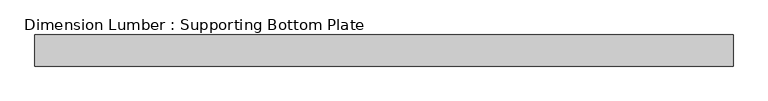
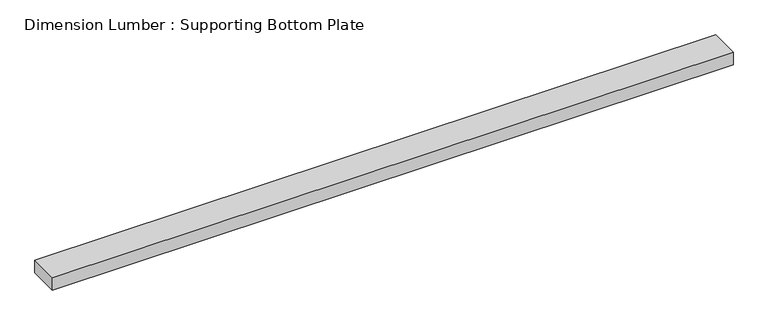
"""IFC4 building model written with IfcOpenShell, lengths in millimetres: beam geometry, Dimension Lumber : Supporting Bottom Plate."""

from ifc_helpers import new_model, si_unit, frame, origin, place, context, project, spatial, polyline, outline, extrude, source, transform, mapped, element, save


def dimension_lumber_supporting_bottom_plate_bb9f9100(model_context):
    return source(origin(), model_context, "Body", "SweptSolid", [
        extrude(outline(polyline([(995.3625, 44.45), (995.3625, -44.45), (-995.3625, -44.45), (-995.3625, 44.45), (995.3625, 44.45)])), frame((0.0, 0.0, -19.05), z_axis=(0.0, 0.0, 1.0), x_axis=(1.0, 0.0, 0.0)), (0.0, 0.0, 1.0), 38.1),
    ])


if __name__ == "__main__":
    model = new_model("IFC4")
    model_context = context("Model", 3, world=origin())
    ifc_project = project(units=[si_unit("LENGTHUNIT", "METRE", prefix="MILLI")], contexts=[model_context])
    site = spatial("IfcSite", under=ifc_project)
    building = spatial("IfcBuilding", under=site)
    placement = place(None, origin())
    dimension_lumber_supporting_bottom_plate_shape = dimension_lumber_supporting_bottom_plate_bb9f9100(model_context)
    element("IfcBeam", 1, ObjectType="Dimension Lumber : Supporting Bottom Plate", at=placement, inside=building, context=model_context, shape_type="MappedRepresentation", body=[
        mapped(dimension_lumber_supporting_bottom_plate_shape, transform((0.0, 0.0, 0.0), x_axis=(1.0, 0.0, 0.0), y_axis=(0.0, 1.0, 0.0), z_axis=(0.0, 0.0, 1.0))),
    ])
    save(model, "model.ifc")

# Revit data of these elements
# Type "Dimension Lumber : Supporting Bottom Plate"
#   Assembly Code = "B10"
#   A = 0.0364583 SF
#   Length [instance default] = 5' - 0"
#   b = 0' - 3 1/2"
#   d = 0' - 1 1/2"
#   Structural Material [instance default] = Softwood, Lumber
# Element 1 (IfcBeam, "Dimension Lumber : Supporting Bottom Plate")
#   Structural Material = Douglas Fir #2
#   Materials on its faces: "Douglas Fir #2"
# Materials
#   "Softwood, Lumber": class "Wood", colour RGB 223 192 134, transparency 0, Description = "Pinus Echinata", Cost = 0
#   "Douglas Fir #2": class "Wood", colour RGB 223 192 134, transparency 0, Description = "Pinus Echinata", Cost = 0
